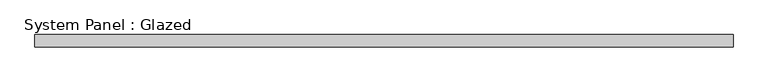
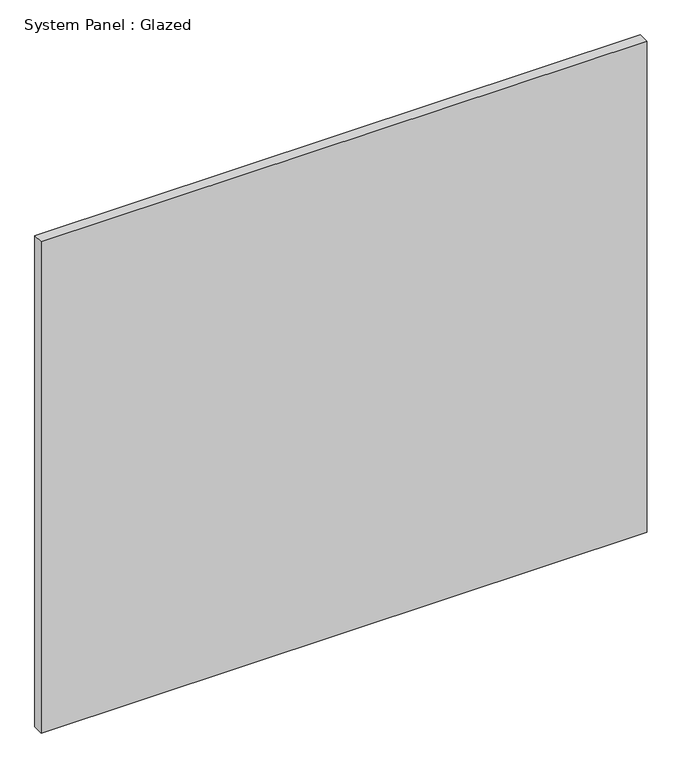
"""IFC4 building model written with IfcOpenShell, lengths in millimetres: plate geometry, System Panel : Glazed."""

from ifc_helpers import new_model, si_unit, origin, origin_with_axes, place, context, project, spatial, polyline, outline, extrude, source, transform, mapped, element, save


def system_panel_glazed_42eec186(model_context):
    return source(origin(), model_context, "Body", "SweptSolid", [
        extrude(outline(polyline([(699.9999998, 24.5), (-699.9999998, 24.5), (-699.9999998, 49.5), (699.9999998, 49.5), (699.9999998, 24.5)])), origin_with_axes(), (0.0, 0.0, 1.0), 1200.0),
    ])


if __name__ == "__main__":
    model = new_model("IFC4")
    model_context = context("Model", 3, world=origin())
    ifc_project = project(units=[si_unit("LENGTHUNIT", "METRE", prefix="MILLI")], contexts=[model_context])
    site = spatial("IfcSite", under=ifc_project)
    building = spatial("IfcBuilding", under=site)
    placement = place(None, origin())
    system_panel_glazed_shape = system_panel_glazed_42eec186(model_context)
    element("IfcPlate", 1, ObjectType="System Panel : Glazed", at=placement, inside=building, context=model_context, shape_type="MappedRepresentation", body=[
        mapped(system_panel_glazed_shape, transform((0.0, 0.0, 0.0), x_axis=(1.0, 0.0, 0.0), y_axis=(0.0, 1.0, 0.0), z_axis=(0.0, 0.0, 1.0))),
    ])
    save(model, "model.ifc")

# Revit data of these elements
# Element 1 (IfcPlate, "System Panel : Glazed")
#   Materials on its faces: "Glass"
# Materials
#   "Glass": class "Glass", colour RGB 218 227 224, transparency 0.85, Description = "Soda Lime Glass", Cost = 0
